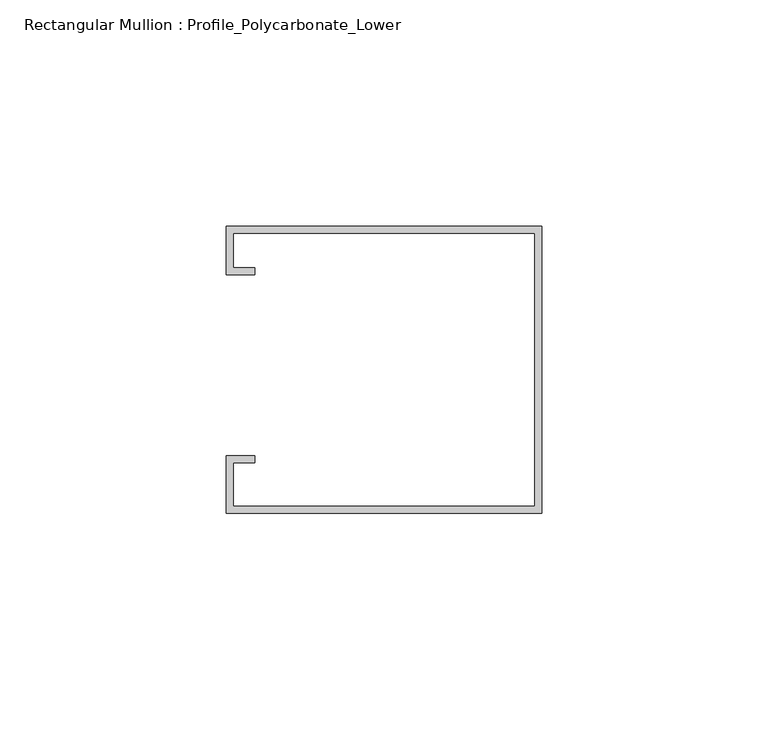
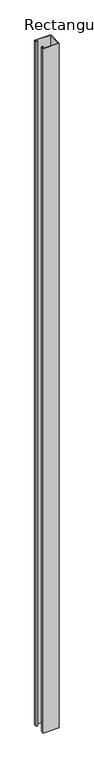
"""IFC4 building model written with IfcOpenShell, lengths in millimetres: member geometry, Rectangular Mullion : Profile_Polycarbonate_Lower."""

from ifc_helpers import new_model, si_unit, frame, origin, place, context, project, spatial, polyline, outline, extrude, source, transform, mapped, element, save


def rectangular_mullion_profile_polycarbonate_lower_e256f0d7(model_context):
    return source(origin(), model_context, "Body", "SweptSolid", [
        extrude(outline(polyline([(0.0, -32.7), (-69.85, -32.7), (-69.85, -20.0), (-63.5, -20.0), (-63.5, -21.5875), (-68.2625, -21.5875), (-68.2625, -31.1125), (-1.5875, -31.1125), (-1.5875, 29.2125), (-68.2625, 29.2125), (-68.2625, 21.5875), (-63.5, 21.5875), (-63.5, 20.0), (-69.85, 20.0), (-69.85, 30.8), (0.0, 30.8), (0.0, -32.7)])), frame((0.0, 0.0, -3136.9), z_axis=(0.0, 0.0, 1.0), x_axis=(1.0, 0.0, 0.0)), (0.0, 0.0, 1.0), 3136.9),
    ])


if __name__ == "__main__":
    model = new_model("IFC4")
    model_context = context("Model", 3, world=origin())
    ifc_project = project(units=[si_unit("LENGTHUNIT", "METRE", prefix="MILLI")], contexts=[model_context])
    site = spatial("IfcSite", under=ifc_project)
    building = spatial("IfcBuilding", under=site)
    placement = place(None, origin())
    rectangular_mullion_profile_polycarbonate_lower_shape = rectangular_mullion_profile_polycarbonate_lower_e256f0d7(model_context)
    element("IfcMember", 1, ObjectType="Rectangular Mullion : Profile_Polycarbonate_Lower", at=placement, inside=building, context=model_context, shape_type="MappedRepresentation", body=[
        mapped(rectangular_mullion_profile_polycarbonate_lower_shape, transform((0.0, 0.0, 0.0), x_axis=(1.0, 0.0, 0.0), y_axis=(0.0, 1.0, 0.0), z_axis=(0.0, 0.0, 1.0))),
    ])
    save(model, "model.ifc")

# Revit data of these elements
# Type "Rectangular Mullion : Profile_Polycarbonate_Lower"
#   built-in parameter 1007322 = 0.208333 (stored number, unit not read)
#   built-in parameter 1007321 = 0 (stored number, unit not read)
#   built-in parameter 1007320 = 0.00520833 (stored number, unit not read)
# Element 1 (IfcMember, "Rectangular Mullion : Profile_Polycarbonate_Lower")
#   Materials on its faces: "ALUMINUM PROFILE AT POLYCARBONATE PANEL"
# Materials
#   "ALUMINUM PROFILE AT POLYCARBONATE PANEL": class "Metal", colour RGB 244 244 244, transparency 0, Description = "Aluminum 6061", Cost = 0
